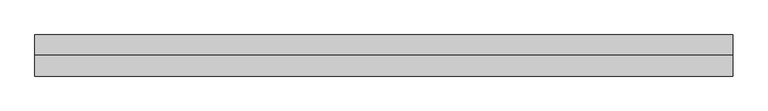
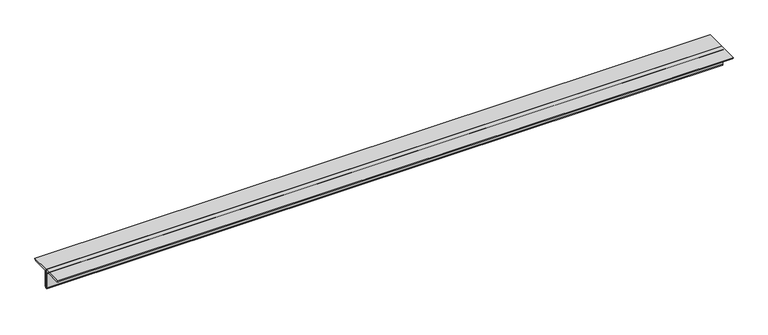
"""IFC4 building model written with IfcOpenShell, lengths in millimetres: member geometry, 0123_Steel Framing_2Ls-KSD3502 : H_SB_AR_S03_2Ls-130x130x12_HBR1."""

import ifcopenshell
import ifcopenshell.guid

model = None  # the IFC model being written
_history = None  # IfcOwnerHistory: only IFC2X3 demands one
_inside = {}  # id of a spatial element -> (the spatial element, [elements in it])
_under = {}  # id of a project, library or spatial element -> (it, [spatial elements below it])
_declared = {}  # id of a project -> (the project, [libraries it declares])
_typed = {}  # id of a type object -> (the type object, [elements of that type])
_made_of = {}  # id of a material, layer set ... -> (it, [elements and type objects made of it])


def new_model(schema):
    """Start an empty IFC model of exactly this schema.

    Asked for "IFC4X3", IfcOpenShell would pick the latest addendum, in which some entities
    have other attributes; the version numbers below select the first issue.
    IFC2X3 requires an IfcOwnerHistory on every rooted entity: one is made here for all.
    """
    global model, _history
    if schema == "IFC4X3":
        model = ifcopenshell.file(schema_version=(4, 3, 0, 0))
    else:
        model = ifcopenshell.file(schema=schema)
    _inside.clear()
    _under.clear()
    _declared.clear()
    _typed.clear()
    _made_of.clear()
    _history = None
    if model.schema == "IFC2X3":
        org = make("IfcOrganization", Name="unknown")
        user = make(
            "IfcPersonAndOrganization",
            ThePerson=make("IfcPerson", FamilyName="unknown"),
            TheOrganization=org,
        )
        app = make(
            "IfcApplication",
            ApplicationDeveloper=org,
            Version="unknown",
            ApplicationFullName="unknown",
            ApplicationIdentifier="unknown",
        )
        _history = make(
            "IfcOwnerHistory",
            OwningUser=user,
            OwningApplication=app,
            ChangeAction="ADDED",
            CreationDate=0,
        )
    return model


def make(cls, **values):
    """One entity of the class cls with the attributes given. An attribute that is None is left unset."""
    return model.create_entity(
        cls, **{name: value for name, value in values.items() if value is not None}
    )


def rooted(cls, **values):
    """An entity with a GlobalId (a new one), such as an element, a storey or a relation."""
    return make(cls, GlobalId=ifcopenshell.guid.new(), OwnerHistory=_history, **values)


def si_unit(unit_type, name, prefix=None):
    """IfcSIUnit, for example si_unit("LENGTHUNIT", "METRE", prefix="MILLI")."""
    return make("IfcSIUnit", UnitType=unit_type, Prefix=prefix, Name=name)


def assignment(units):
    """IfcUnitAssignment: the units of a project."""
    return None if units is None else make("IfcUnitAssignment", Units=units)


def point(xyz):
    """IfcCartesianPoint."""
    return None if xyz is None else make("IfcCartesianPoint", Coordinates=xyz)


def direction(xyz):
    """IfcDirection."""
    return None if xyz is None else make("IfcDirection", DirectionRatios=xyz)


def frame(location, z_axis=None, x_axis=None):
    """IfcAxis2Placement3D, a coordinate frame: its origin and axes. An axis left out is left unset."""
    return make(
        "IfcAxis2Placement3D",
        Location=point(location),
        Axis=direction(z_axis),
        RefDirection=direction(x_axis),
    )


def frame_2d(location, x_axis=None):
    """IfcAxis2Placement2D, a coordinate frame in the plane: its origin and x axis."""
    return make(
        "IfcAxis2Placement2D", Location=point(location), RefDirection=direction(x_axis)
    )


def origin():
    """The frame at (0, 0, 0) with its axes left unset."""
    return frame((0.0, 0.0, 0.0))


def place(relative_to, where):
    """IfcLocalPlacement: puts the frame where relative to a parent placement (None: the world)."""
    return make(
        "IfcLocalPlacement", PlacementRelTo=relative_to, RelativePlacement=where
    )


def context(
    kind, dimensions, precision=None, world=None, true_north=None, identifier=None
):
    """IfcGeometricRepresentationContext, for example the 3D "Model" context."""
    return make(
        "IfcGeometricRepresentationContext",
        ContextIdentifier=identifier,
        ContextType=kind,
        CoordinateSpaceDimension=dimensions,
        Precision=precision,
        WorldCoordinateSystem=world,
        TrueNorth=true_north,
    )


def project(units=None, contexts=None):
    """IfcProject with its units and contexts."""
    return rooted(
        "IfcProject",
        Name="project",
        RepresentationContexts=contexts,
        UnitsInContext=assignment(units),
    )


def spatial(cls, under=None, at=None, **own):
    """A site, building, storey or space (cls), placed at a placement, below another one or the project."""
    s = rooted(cls, ObjectPlacement=at, **own)
    if under is not None:
        _under.setdefault(under.id(), (under, []))[1].append(s)
    return s


def polyline(points):
    """IfcPolyline through the points."""
    return make("IfcPolyline", Points=[point(p) for p in points])


def circle_curve(where, radius):
    """IfcCircle in the frame where."""
    return make("IfcCircle", Position=where, Radius=radius)


def trimmed(basis, trim1, trim2, sense, master):
    """IfcTrimmedCurve: the piece of a basis curve between two trims."""
    return make(
        "IfcTrimmedCurve",
        BasisCurve=basis,
        Trim1=trim1,
        Trim2=trim2,
        SenseAgreement=sense,
        MasterRepresentation=master,
    )


def segment(curve, same_sense, transition):
    """IfcCompositeCurveSegment."""
    return make(
        "IfcCompositeCurveSegment",
        Transition=transition,
        SameSense=same_sense,
        ParentCurve=curve,
    )


def composite_curve(segments, self_intersect=None):
    """IfcCompositeCurve: segments joined end to end."""
    return make("IfcCompositeCurve", Segments=segments, SelfIntersect=self_intersect)


def outline(outer, holes=None, kind="AREA"):
    """IfcArbitraryClosedProfileDef: a profile drawn as a closed curve; with holes, ...WithVoids."""
    if holes is None:
        return make("IfcArbitraryClosedProfileDef", ProfileType=kind, OuterCurve=outer)
    return make(
        "IfcArbitraryProfileDefWithVoids",
        ProfileType=kind,
        OuterCurve=outer,
        InnerCurves=holes,
    )


def extrude(swept, where, along, depth):
    """IfcExtrudedAreaSolid: the profile swept, set in the frame where, extruded along a direction by depth."""
    return make(
        "IfcExtrudedAreaSolid",
        SweptArea=swept,
        Position=where,
        ExtrudedDirection=direction(along),
        Depth=depth,
    )


def shape(context_of_items, identifier, shape_type, items):
    """IfcShapeRepresentation: the items that make up one representation, for example the "Body"."""
    return make(
        "IfcShapeRepresentation",
        ContextOfItems=context_of_items,
        RepresentationIdentifier=identifier,
        RepresentationType=shape_type,
        Items=items,
    )


def source(mapping_origin, context_of_items, identifier, shape_type, items):
    """IfcRepresentationMap: a shape defined once, which mapped items show again and again."""
    return make(
        "IfcRepresentationMap",
        MappingOrigin=mapping_origin,
        MappedRepresentation=shape(context_of_items, identifier, shape_type, items),
    )


def transform(
    local_origin,
    x_axis=None,
    y_axis=None,
    z_axis=None,
    scale=None,
    scale2=None,
    scale3=None,
    uniform=True,
):
    """IfcCartesianTransformationOperator3D, or its non-uniform kind. x_axis, y_axis, z_axis: its Axis1, 2, 3."""
    if uniform:
        return make(
            "IfcCartesianTransformationOperator3D",
            Axis1=direction(x_axis),
            Axis2=direction(y_axis),
            LocalOrigin=point(local_origin),
            Scale=scale,
            Axis3=direction(z_axis),
        )
    return make(
        "IfcCartesianTransformationOperator3DnonUniform",
        Axis1=direction(x_axis),
        Axis2=direction(y_axis),
        LocalOrigin=point(local_origin),
        Scale=scale,
        Axis3=direction(z_axis),
        Scale2=scale2,
        Scale3=scale3,
    )


def mapped(mapping_source, mapping_target):
    """IfcMappedItem: shows the shape of a source again, moved by a transform."""
    return make(
        "IfcMappedItem", MappingSource=mapping_source, MappingTarget=mapping_target
    )


def made_of(thing, what):
    """Note that an element or type object is made of a material, layer set ...; save() writes the relation."""
    if what is not None:
        _made_of.setdefault(what.id(), (what, []))[1].append(thing)
    return thing


def element(
    cls,
    number,
    at=None,
    inside=None,
    cuts=None,
    type_object=None,
    material=None,
    context=None,
    identifier="Body",
    shape_type=None,
    held_by="IfcProductDefinitionShape",
    body=None,
    shapes=None,
    **own,
):
    """One element of the class cls, such as IfcWall. Its Tag is "e" and its number.

    at: its placement. inside: the storey or other place that contains it. cuts: it is an
    opening in that element (IfcRelVoidsElement). A single representation is given by context,
    identifier, shape_type and body (its items); several are given by shapes. held_by: the class
    of the entity that holds the representations. save() writes the other relations.
    """
    e = rooted(cls, Tag="e%d" % number, ObjectPlacement=at, **own)
    if body is not None:
        shapes = [shape(context, identifier, shape_type, body)]
    if shapes is not None:
        e.Representation = make(held_by, Representations=shapes)
    if inside is not None:
        _inside.setdefault(inside.id(), (inside, []))[1].append(e)
    if cuts is not None:
        rooted(
            "IfcRelVoidsElement", RelatingBuildingElement=cuts, RelatedOpeningElement=e
        )
    if type_object is not None:
        _typed.setdefault(type_object.id(), (type_object, []))[1].append(e)
    return made_of(e, material)


def aggregate(whole, parts):
    """IfcRelAggregates: a whole, such as a stair, and the parts it consists of."""
    return rooted("IfcRelAggregates", RelatingObject=whole, RelatedObjects=parts)


def save(model, path):
    """Write the relations noted so far, then the file.

    IfcRelAggregates (storeys below a building ...), IfcRelContainedInSpatialStructure (elements
    in a storey), IfcRelDefinesByType, IfcRelAssociatesMaterial and IfcRelDeclares: one each for
    every whole, place, type object, material and project.
    """
    for whole, parts in _under.values():
        aggregate(whole, parts)
    for where, things in _inside.values():
        rooted(
            "IfcRelContainedInSpatialStructure",
            RelatedElements=things,
            RelatingStructure=where,
        )
    for kind, things in _typed.values():
        rooted("IfcRelDefinesByType", RelatedObjects=things, RelatingType=kind)
    for what, things in _made_of.values():
        rooted("IfcRelAssociatesMaterial", RelatedObjects=things, RelatingMaterial=what)
    for by, libraries in _declared.values():
        rooted("IfcRelDeclares", RelatingContext=by, RelatedDefinitions=libraries)
    model.write(path)


def member_7318b5d7(model_context):
    return source(origin(), model_context, "Body", "SweptSolid", [
        extrude(outline(composite_curve([segment(polyline([(0.0, 36.4), (0.0, -93.6)]), True, "CONTINUOUS"), segment(trimmed(circle_curve(frame_2d((0.0, -81.6)), 12.0), [point((0.0, -93.6))], [point((-12.0, -81.6))], False, "CARTESIAN"), True, "CONTINUOUS"), segment(polyline([(-12.0, -81.6), (-12.0, 12.4)]), True, "CONTINUOUS"), segment(trimmed(circle_curve(frame_2d((-24.0, 12.4)), 12.0), [point((-12.0, 12.4))], [point((-24.0, 24.4))], True, "CARTESIAN"), True, "CONTINUOUS"), segment(polyline([(-24.0, 24.4), (-118.0, 24.4)]), True, "CONTINUOUS"), segment(trimmed(circle_curve(frame_2d((-118.0, 36.4)), 12.0), [point((-118.0, 24.4))], [point((-130.0, 36.4))], False, "CARTESIAN"), True, "CONTINUOUS"), segment(polyline([(-130.0, 36.4), (0.0, 36.4)]), True, "CONTINUOUS")], self_intersect=False)), frame((-2254.4342987, 0.0, 0.0), z_axis=(1.0, 0.0, 0.0), x_axis=(0.0, 1.0, 0.0)), (0.0, 0.0, 1.0), 4412.2019305),
        extrude(outline(composite_curve([segment(polyline([(0.0, 36.4), (130.0, 36.4)]), True, "CONTINUOUS"), segment(trimmed(circle_curve(frame_2d((118.0, 36.4)), 12.0), [point((130.0, 36.4))], [point((118.0, 24.4))], False, "CARTESIAN"), True, "CONTINUOUS"), segment(polyline([(118.0, 24.4), (24.0, 24.4)]), True, "CONTINUOUS"), segment(trimmed(circle_curve(frame_2d((24.0, 12.4)), 12.0), [point((24.0, 24.4))], [point((12.0, 12.4))], True, "CARTESIAN"), True, "CONTINUOUS"), segment(polyline([(12.0, 12.4), (12.0, -81.6)]), True, "CONTINUOUS"), segment(trimmed(circle_curve(frame_2d((0.0, -81.6)), 12.0), [point((12.0, -81.6))], [point((0.0, -93.6))], False, "CARTESIAN"), True, "CONTINUOUS"), segment(polyline([(0.0, -93.6), (0.0, 36.4)]), True, "CONTINUOUS")], self_intersect=False)), frame((-2254.4342987, 0.0, 0.0), z_axis=(1.0, 0.0, 0.0), x_axis=(0.0, 1.0, 0.0)), (0.0, 0.0, 1.0), 4412.2019305),
    ])


if __name__ == "__main__":
    model = new_model("IFC4")
    model_context = context("Model", 3, world=origin())
    ifc_project = project(units=[si_unit("LENGTHUNIT", "METRE", prefix="MILLI")], contexts=[model_context])
    site = spatial("IfcSite", under=ifc_project)
    building = spatial("IfcBuilding", under=site)
    placement = place(None, origin())
    member_shape = member_7318b5d7(model_context)
    element("IfcMember", 1, ObjectType="0123_Steel Framing_2Ls-KSD3502 : H_SB_AR_S03_2Ls-130x130x12_HBR1", at=placement, inside=building, context=model_context, shape_type="MappedRepresentation", body=[
        mapped(member_shape, transform((0.0, 0.0, 0.0), x_axis=(1.0, 0.0, 0.0), y_axis=(0.0, 1.0, 0.0), z_axis=(0.0, 0.0, 1.0))),
    ])
    save(model, "model.ifc")

# Revit data of these elements
# Type "0123_Steel Framing_2Ls-KSD3502 : H_SB_AR_S03_2Ls-130x130x12_HBR1"
#   Assembly Code = "B10"
#   Legs = "SLBB"
#   W = 8.97
#   Perimeter = 1.04 m²/m
#   Nominal Weight = 46.80 kgf/m
#   Length [instance default] = 1000 mm
#   Space = 0 mm
#   b = 130 mm
#   d = 130 mm
#   t = 12 mm
#   y = 36.4 mm
#   A = 0.005952 m²
#   Structural Material [instance default] = Steel ASTM A36
# Element 1 (IfcMember, "0123_Steel Framing_2Ls-KSD3502 : H_SB_AR_S03_2Ls-130x130x12_HBR1")
#   Structural Material = Steel, 45-345
#   Materials on its faces: "Steel, 45-345"
# Materials
#   "Steel ASTM A36": class "Metal", colour RGB 199 199 199, transparency 0, Description = "Structural steel, ASTM A36 Grade B, mill finish", Cost = 0
#   "Steel, 45-345": class "Metal", colour RGB 189 187 185, transparency 0, Description = "Steel 345 MPa", Cost = 0
